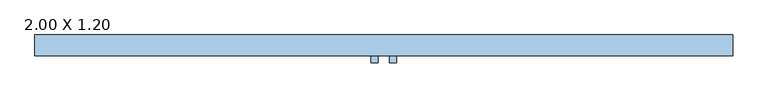
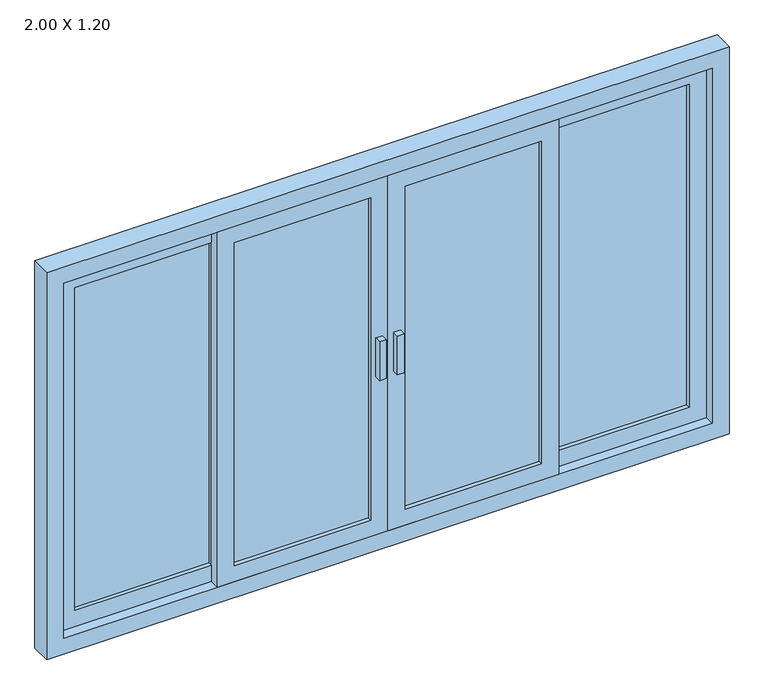
"""IFC4 building model written with IfcOpenShell, lengths in millimetres: window geometry, JANELA_DE_CORRER_4 FOLHAS_VIDRO : 2.00 X 1.20."""

from ifc_helpers import new_model, si_unit, frame, origin, place, context, project, spatial, polyline, outline, extrude, source, transform, mapped, element, save


def window_2_00_x_1_20_22b3e67b(model_context):
    return source(origin(), model_context, "Body", "SweptSolid", [
        extrude(outline(polyline([(900.0, 17.5), (900.0, 12.5), (500.0, 12.5), (500.0, 17.5), (900.0, 17.5)])), frame((0.0, 0.0, 1100.0), z_axis=(0.0, 0.0, 1.0), x_axis=(1.0, 0.0, 0.0)), (0.0, 0.0, 1.0), 1000.0),
        extrude(outline(polyline([(2150.0, 950.0), (2150.0, 450.0), (1050.0, 450.0), (1050.0, 950.0), (2150.0, 950.0)]), holes=[polyline([(2100.0, 900.0), (1100.0, 900.0), (1100.0, 500.0), (2100.0, 500.0), (2100.0, 900.0)])]), frame((0.0, 0.0, 0.0), z_axis=(0.0, 1.0, 0.0), x_axis=(0.0, 0.0, 1.0)), (0.0, 0.0, 1.0), 30.0),
        extrude(outline(polyline([(450.0, -12.5), (450.0, -17.5), (50.0, -17.5), (50.0, -12.5), (450.0, -12.5)])), frame((0.0, 0.0, 1100.0), z_axis=(0.0, 0.0, 1.0), x_axis=(1.0, 0.0, 0.0)), (0.0, 0.0, 1.0), 1000.0),
        extrude(outline(polyline([(2150.0, 500.0), (2150.0, 0.0), (1050.0, 0.0), (1050.0, 500.0), (2150.0, 500.0)]), holes=[polyline([(2100.0, 450.0), (1100.0, 450.0), (1100.0, 50.0), (2100.0, 50.0), (2100.0, 450.0)])]), frame((0.0, -30.0, 0.0), z_axis=(0.0, 1.0, 0.0), x_axis=(0.0, 0.0, 1.0)), (0.0, 0.0, 1.0), 30.0),
        extrude(outline(polyline([(-50.0, -12.5), (-50.0, -17.5), (-450.0, -17.5), (-450.0, -12.5), (-50.0, -12.5)])), frame((0.0, 0.0, 1100.0), z_axis=(0.0, 0.0, 1.0), x_axis=(1.0, 0.0, 0.0)), (0.0, 0.0, 1.0), 1000.0),
        extrude(outline(polyline([(2150.0, 0.0), (2150.0, -500.0), (1050.0, -500.0), (1050.0, 0.0), (2150.0, 0.0)]), holes=[polyline([(2100.0, -50.0), (1100.0, -50.0), (1100.0, -450.0), (2100.0, -450.0), (2100.0, -50.0)])]), frame((0.0, -30.0, 0.0), z_axis=(0.0, 1.0, 0.0), x_axis=(0.0, 0.0, 1.0)), (0.0, 0.0, 1.0), 30.0),
        extrude(outline(polyline([(-500.0, 17.5), (-500.0, 12.5), (-900.0, 12.5), (-900.0, 17.5), (-500.0, 17.5)])), frame((0.0, 0.0, 1100.0), z_axis=(0.0, 0.0, 1.0), x_axis=(1.0, 0.0, 0.0)), (0.0, 0.0, 1.0), 1000.0),
        extrude(outline(polyline([(2150.0, -450.0), (2150.0, -950.0), (1050.0, -950.0), (1050.0, -450.0), (2150.0, -450.0)]), holes=[polyline([(2100.0, -500.0), (1100.0, -500.0), (1100.0, -900.0), (2100.0, -900.0), (2100.0, -500.0)])]), frame((0.0, 0.0, 0.0), z_axis=(0.0, 1.0, 0.0), x_axis=(0.0, 0.0, 1.0)), (0.0, 0.0, 1.0), 30.0),
        extrude(outline(polyline([(1000.0, -1000.0), (1000.0, 1000.0), (2200.0, 1000.0), (2200.0, -1000.0), (1000.0, -1000.0)]), holes=[polyline([(2150.0, -950.0), (2150.0, 950.0), (1050.0, 950.0), (1050.0, -950.0), (2150.0, -950.0)])]), frame((0.0, -30.0, 0.0), z_axis=(0.0, 1.0, 0.0), x_axis=(0.0, 0.0, 1.0)), (0.0, 0.0, 1.0), 60.0),
        extrude(outline(polyline([(15.9492003, -30.0), (35.9492003, -30.0), (35.9492003, -50.0), (15.9492003, -50.0), (15.9492003, -30.0)])), frame((0.0, 0.0, 1540.0), z_axis=(0.0, 0.0, 1.0), x_axis=(1.0, 0.0, 0.0)), (0.0, 0.0, 1.0), 120.0),
        extrude(outline(polyline([(-35.9492003, -30.0), (-15.9492003, -30.0), (-15.9492003, -50.0), (-35.9492003, -50.0), (-35.9492003, -30.0)])), frame((0.0, 0.0, 1540.0), z_axis=(0.0, 0.0, 1.0), x_axis=(1.0, 0.0, 0.0)), (0.0, 0.0, 1.0), 120.0),
    ])


if __name__ == "__main__":
    model = new_model("IFC4")
    model_context = context("Model", 3, world=origin())
    ifc_project = project(units=[si_unit("LENGTHUNIT", "METRE", prefix="MILLI")], contexts=[model_context])
    site = spatial("IfcSite", under=ifc_project)
    building = spatial("IfcBuilding", under=site)
    placement = place(None, origin())
    window_2_00_x_1_20_shape = window_2_00_x_1_20_22b3e67b(model_context)
    element("IfcWindow", 1, ObjectType="JANELA_DE_CORRER_4 FOLHAS_VIDRO : 2.00 X 1.20", at=placement, inside=building, context=model_context, shape_type="MappedRepresentation", body=[
        mapped(window_2_00_x_1_20_shape, transform((0.0, 0.0, 0.0), x_axis=(1.0, 0.0, 0.0), y_axis=(0.0, 1.0, 0.0), z_axis=(0.0, 0.0, 1.0))),
    ])
    save(model, "model.ifc")

# Revit data of these elements
# Type "JANELA_DE_CORRER_4 FOLHAS_VIDRO : 2.00 X 1.20"
#   Type Mark = "J1"
#   Analytic Construction = "<Nenhum>"
#   Largura moldura = 0.06 m
#   Largura janela = 1.90 m
#   Largura esquadria = 0.05 m
#   Largura do painel = 0.50 m
#   Largura da moldura do painel = 0.05 m
#   Espessura painel = 0.03 m
#   Espessura moldura = 0.03 m
#   Altura janela = 1.10 m
#   Height = 1.20 m
#   Altura-padrão do peitoril = 1.00 m
#   Width = 2.00 m
#   Puxadores [instance default] = yes
#   Moldura interna [instance default] = yes
#   Moldura externa [instance default] = yes
#   Tipo de vidro = .VIDRO
#   Material puxadores = .ALUMÍNIO COM PINTURA ELETROSTÁTICA BRANCA
#   Material moldura = .ALUMÍNIO COM PINTURA ELETROSTÁTICA BRANCA
#   Material da esquadria = .ALUMÍNIO COM PINTURA ELETROSTÁTICA BRANCA
#   Wall Closure = (empty or 0)
# Element 1 (IfcWindow, "JANELA_DE_CORRER_4 FOLHAS_VIDRO : 2.00 X 1.20")
#   Moldura interna = no
#   Moldura externa = no
#   Materials on its faces: ".ALUMÍNIO COM PINTURA ELETROSTÁTICA BRANCA", ".VIDRO"
# Materials
#   ".VIDRO": class "Genérico", colour RGB 198 236 255, transparency 0.95, Cost = 0
#   ".ALUMÍNIO COM PINTURA ELETROSTÁTICA BRANCA": class "CC_METAIS", colour RGB 241 241 241, transparency 0, Cost = 0
